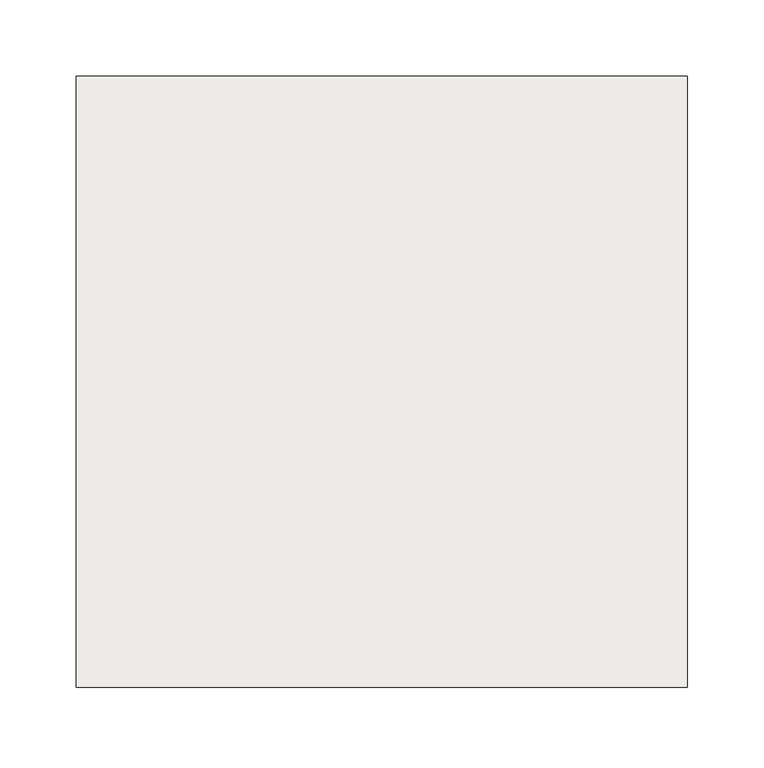
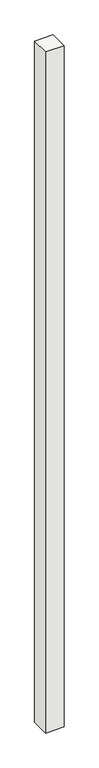
"""IFC4 building model written with IfcOpenShell, lengths in millimetres: slab geometry, NLRS_17_SFO_TLB_funderingspaal geheid beton prefab-AV-MMBPC_gen_rsf : heipaal beton prefab_gen__bxh 400x400."""

from ifc_helpers import new_model, si_unit, frame, origin, place, context, project, spatial, polyline, outline, extrude, source, transform, mapped, element, save


def slab_4eaa82be(model_context):
    return source(origin(), model_context, "Body", "SweptSolid", [
        extrude(outline(polyline([(200.0, -200.0), (-200.0, -200.0), (-200.0, 200.0), (200.0, 200.0), (200.0, -200.0)])), frame((0.0, 0.0, -20000.0), z_axis=(0.0, 0.0, 1.0), x_axis=(1.0, 0.0, 0.0)), (0.0, 0.0, 1.0), 15520.0),
    ])


if __name__ == "__main__":
    model = new_model("IFC4")
    model_context = context("Model", 3, world=origin())
    ifc_project = project(units=[si_unit("LENGTHUNIT", "METRE", prefix="MILLI")], contexts=[model_context])
    site = spatial("IfcSite", under=ifc_project)
    building = spatial("IfcBuilding", under=site)
    placement = place(None, origin())
    slab_shape = slab_4eaa82be(model_context)
    element("IfcSlab", 1, ObjectType="NLRS_17_SFO_TLB_funderingspaal geheid beton prefab-AV-MMBPC_gen_rsf : heipaal beton prefab_gen__bxh 400x400", at=placement, inside=building, context=model_context, shape_type="MappedRepresentation", body=[
        mapped(slab_shape, transform((0.0, 0.0, 0.0), x_axis=(1.0, 0.0, 0.0), y_axis=(0.0, 1.0, 0.0), z_axis=(0.0, 0.0, 1.0))),
    ])
    save(model, "model.ifc")

# Revit data of these elements
# Type "NLRS_17_SFO_TLB_funderingspaal geheid beton prefab-AV-MMBPC_gen_rsf : heipaal beton prefab_gen__bxh 400x400"
#   Export Type to IFC As = "IfcPile"
#   Type IfcGUID = "10$Kfo5uPCAOPJEOo5LE_W"
#   Type Comments = "prefab heipaal 400x400"
#   Model = " "
#   Manufacturer = " "
#   Description = "prefab heipaal 400x400"
#   Assembly Code = "17.21"
#   Width = 400 mm
#   Slanted Angle [instance default] = 0.00°
#   NLRS_S_draagvermogen_trek [instance default] = 0.00 kN
#   NLRS_S_draagvermogen_druk [instance default] = 0.00 kN
#   NLRS_C_lengte [instance default] = 1660 mm
#   NLRS_C_hoogte = 400 mm
#   NLRS_C_breedte = 400 mm
#   Height [instance default] = 1660 mm
#   Length [instance default] = 1660 mm
#   Angle [instance default] = 0.00°
#   Slanted [instance default] = 0
#   Structural Material = NLRS_f2_beton prefab_gen_rsf
#   Keynote = ""
# Element 1 (IfcSlab, "NLRS_17_SFO_TLB_funderingspaal geheid beton prefab-AV-MMBPC_gen_rsf : heipaal beton prefab_gen__bxh 400x400")
#   NLRS_C_lengte = 15520 mm
#   Height = 15520 mm
#   Length = 15520 mm
#   Materials on its faces: "NLRS_f2_beton prefab_gen_rsf"
# Materials
#   "NLRS_f2_beton prefab_gen_rsf": class "F - Niet gebakken kunststeen", colour RGB 129 133 118, transparency 0, Keynote = "f2", Manufacturer = "Revit Standards Foundation", URL = "www.revitstandards.org", Description = "beton prefab", Cost = 0
